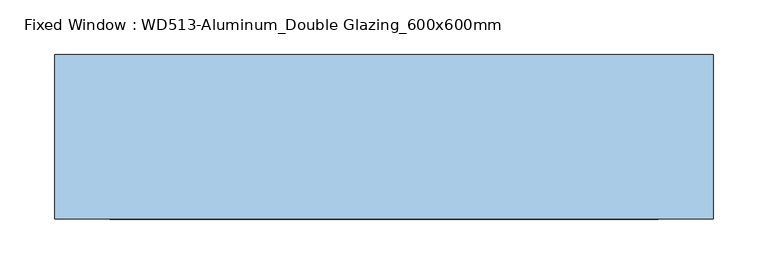
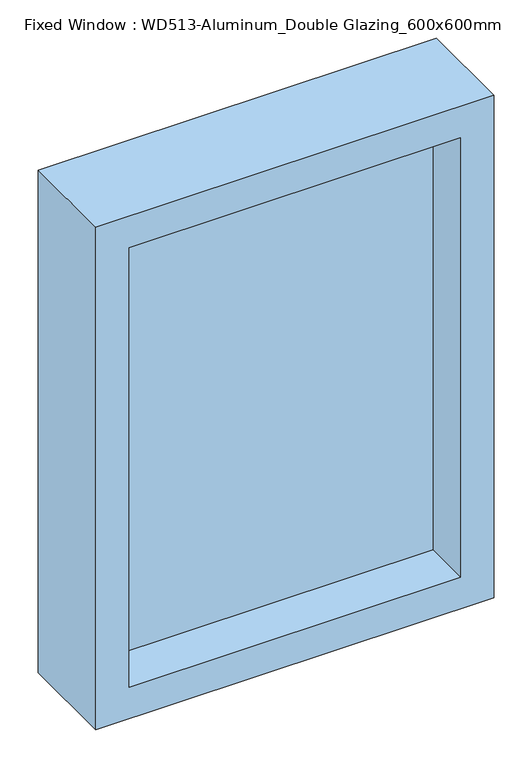
"""IFC4 building model written with IfcOpenShell, lengths in millimetres: window geometry, Fixed Window : WD513-Aluminum_Double Glazing_600x600mm."""

from ifc_helpers import new_model, si_unit, frame, origin, place, context, project, spatial, polyline, outline, extrude, source, transform, mapped, element, save


def fixed_window_wd513_aluminum_double_glazing_600x600mm_37dd25d6(model_context):
    return source(origin(), model_context, "Body", "SweptSolid", [
        extrude(outline(polyline([(-250.0, 3.0), (250.0, 3.0), (250.0, -3.0), (-250.0, -3.0), (-250.0, 3.0)])), frame((0.0, 0.0, 850.0), z_axis=(0.0, 0.0, 1.0), x_axis=(1.0, 0.0, 0.0)), (0.0, 0.0, 1.0), 700.0),
        extrude(outline(polyline([(1600.0, -300.0), (800.0, -300.0), (800.0, 300.0), (1600.0, 300.0), (1600.0, -300.0)]), holes=[polyline([(1550.0, -250.0), (1550.0, 250.0), (850.0, 250.0), (850.0, -250.0), (1550.0, -250.0)])]), frame((0.0, -75.0, 0.0), z_axis=(0.0, 1.0, 0.0), x_axis=(0.0, 0.0, 1.0)), (0.0, 0.0, 1.0), 150.0),
    ])


if __name__ == "__main__":
    model = new_model("IFC4")
    model_context = context("Model", 3, world=origin())
    ifc_project = project(units=[si_unit("LENGTHUNIT", "METRE", prefix="MILLI")], contexts=[model_context])
    site = spatial("IfcSite", under=ifc_project)
    building = spatial("IfcBuilding", under=site)
    placement = place(None, origin())
    fixed_window_wd513_aluminum_double_glazing_600x600mm_shape = fixed_window_wd513_aluminum_double_glazing_600x600mm_37dd25d6(model_context)
    element("IfcWindow", 1, ObjectType="Fixed Window : WD513-Aluminum_Double Glazing_600x600mm", at=placement, inside=building, context=model_context, shape_type="MappedRepresentation", body=[
        mapped(fixed_window_wd513_aluminum_double_glazing_600x600mm_shape, transform((0.0, 0.0, 0.0), x_axis=(1.0, 0.0, 0.0), y_axis=(0.0, 1.0, 0.0), z_axis=(0.0, 0.0, 1.0))),
    ])
    save(model, "model.ifc")

# Revit data of these elements
# Type "Fixed Window : WD513-Aluminum_Double Glazing_600x600mm"
#   Type Mark = "AW"
#   Analytic Construction = "<None>"
#   창 두께 = 150 mm
#   Height = 800 mm
#   절반 창 두께 = 75 mm
#   기본 씰 높이 = 800 mm
#   Width = 600 mm
#   Define Thermal Properties by = 1
#   창 패널 = AW2 창 패널
#   창 프레임 = A04AQ127-00002_Aluminum Window_None FP
#   Wall Closure = (empty or 0)
# Element 1 (IfcWindow, "Fixed Window : WD513-Aluminum_Double Glazing_600x600mm")
#   Materials on its faces: "A04AQ127-00002_Aluminum Window_None FP", "AW2 창 패널"
# Materials
#   "AW2 창 패널": class "유리", colour RGB 0 0 255, transparency 0.75
#   "A04AQ127-00002_Aluminum Window_None FP": class "금속", colour RGB 247 247 247, transparency 0, W00) Work Master Code = "A04AQ127-00002", W01) Work Master_Lv1 = "Finishing Work", W02) Work Master_Lv2 = "Door & Window Work", W03) Work Master_Spec.1 = "Aluminum Window", W04) Work Master_Spec.2 = "Fire Protective Rating: N/A", W05) Work Master_Spec.3 = "w/ Hardware & Accessories", Cost = 0
